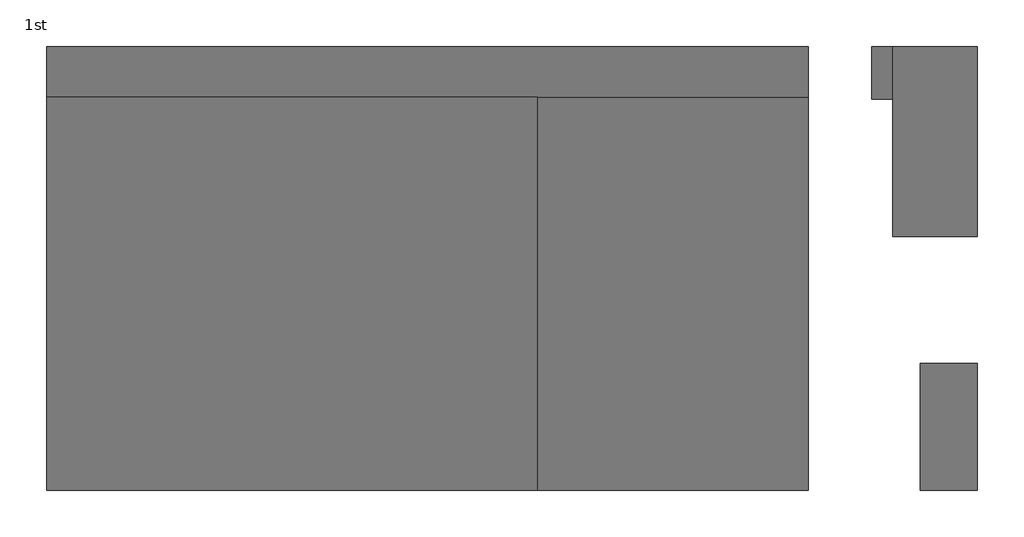
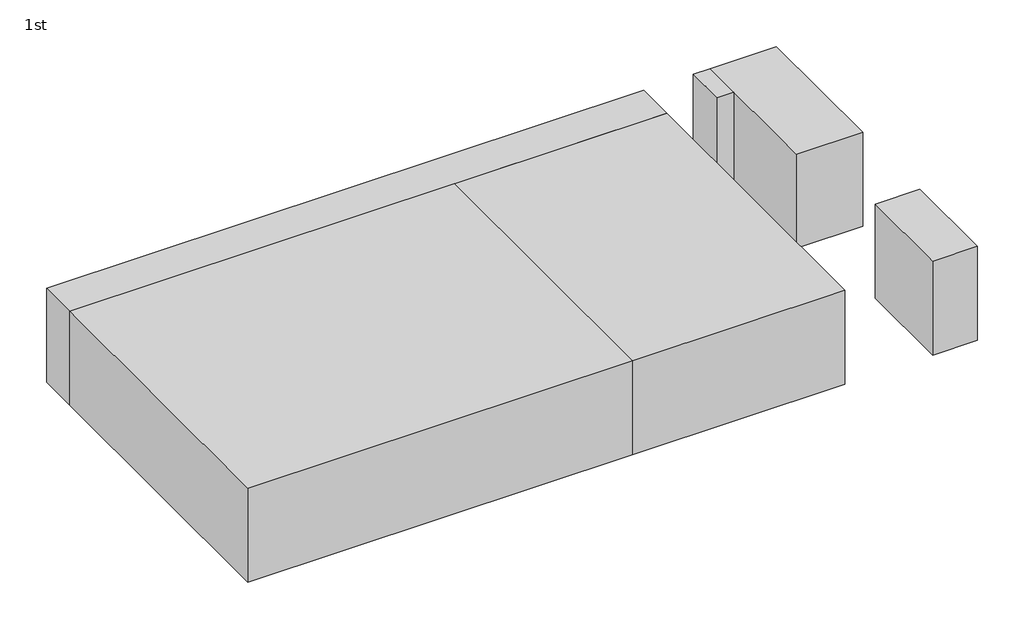
# One storey: 6 proxies.
"""IFC4 building model written with IfcOpenShell, lengths in millimetres."""

import ifcopenshell
import ifcopenshell.guid

model = None  # the IFC model being written
_history = None  # IfcOwnerHistory: only IFC2X3 demands one
_inside = {}  # id of a spatial element -> (the spatial element, [elements in it])
_under = {}  # id of a project, library or spatial element -> (it, [spatial elements below it])
_declared = {}  # id of a project -> (the project, [libraries it declares])
_typed = {}  # id of a type object -> (the type object, [elements of that type])
_made_of = {}  # id of a material, layer set ... -> (it, [elements and type objects made of it])


def new_model(schema):
    """Start an empty IFC model of exactly this schema.

    Asked for "IFC4X3", IfcOpenShell would pick the latest addendum, in which some entities
    have other attributes; the version numbers below select the first issue.
    IFC2X3 requires an IfcOwnerHistory on every rooted entity: one is made here for all.
    """
    global model, _history
    if schema == "IFC4X3":
        model = ifcopenshell.file(schema_version=(4, 3, 0, 0))
    else:
        model = ifcopenshell.file(schema=schema)
    _inside.clear()
    _under.clear()
    _declared.clear()
    _typed.clear()
    _made_of.clear()
    _history = None
    if model.schema == "IFC2X3":
        org = make("IfcOrganization", Name="unknown")
        user = make(
            "IfcPersonAndOrganization",
            ThePerson=make("IfcPerson", FamilyName="unknown"),
            TheOrganization=org,
        )
        app = make(
            "IfcApplication",
            ApplicationDeveloper=org,
            Version="unknown",
            ApplicationFullName="unknown",
            ApplicationIdentifier="unknown",
        )
        _history = make(
            "IfcOwnerHistory",
            OwningUser=user,
            OwningApplication=app,
            ChangeAction="ADDED",
            CreationDate=0,
        )
    return model


def make(cls, **values):
    """One entity of the class cls with the attributes given. An attribute that is None is left unset."""
    return model.create_entity(
        cls, **{name: value for name, value in values.items() if value is not None}
    )


def rooted(cls, **values):
    """An entity with a GlobalId (a new one), such as an element, a storey or a relation."""
    return make(cls, GlobalId=ifcopenshell.guid.new(), OwnerHistory=_history, **values)


def si_unit(unit_type, name, prefix=None):
    """IfcSIUnit, for example si_unit("LENGTHUNIT", "METRE", prefix="MILLI")."""
    return make("IfcSIUnit", UnitType=unit_type, Prefix=prefix, Name=name)


def assignment(units):
    """IfcUnitAssignment: the units of a project."""
    return None if units is None else make("IfcUnitAssignment", Units=units)


def point(xyz):
    """IfcCartesianPoint."""
    return None if xyz is None else make("IfcCartesianPoint", Coordinates=xyz)


def direction(xyz):
    """IfcDirection."""
    return None if xyz is None else make("IfcDirection", DirectionRatios=xyz)


def frame(location, z_axis=None, x_axis=None):
    """IfcAxis2Placement3D, a coordinate frame: its origin and axes. An axis left out is left unset."""
    return make(
        "IfcAxis2Placement3D",
        Location=point(location),
        Axis=direction(z_axis),
        RefDirection=direction(x_axis),
    )


def origin():
    """The frame at (0, 0, 0) with its axes left unset."""
    return frame((0.0, 0.0, 0.0))


def origin_with_axes():
    """The frame at (0, 0, 0) with the z axis (0, 0, 1) and the x axis (1, 0, 0) written out."""
    return frame((0.0, 0.0, 0.0), z_axis=(0.0, 0.0, 1.0), x_axis=(1.0, 0.0, 0.0))


def place(relative_to, where):
    """IfcLocalPlacement: puts the frame where relative to a parent placement (None: the world)."""
    return make(
        "IfcLocalPlacement", PlacementRelTo=relative_to, RelativePlacement=where
    )


def context(
    kind, dimensions, precision=None, world=None, true_north=None, identifier=None
):
    """IfcGeometricRepresentationContext, for example the 3D "Model" context."""
    return make(
        "IfcGeometricRepresentationContext",
        ContextIdentifier=identifier,
        ContextType=kind,
        CoordinateSpaceDimension=dimensions,
        Precision=precision,
        WorldCoordinateSystem=world,
        TrueNorth=true_north,
    )


def project(units=None, contexts=None):
    """IfcProject with its units and contexts."""
    return rooted(
        "IfcProject",
        Name="project",
        RepresentationContexts=contexts,
        UnitsInContext=assignment(units),
    )


def spatial(cls, under=None, at=None, **own):
    """A site, building, storey or space (cls), placed at a placement, below another one or the project."""
    s = rooted(cls, ObjectPlacement=at, **own)
    if under is not None:
        _under.setdefault(under.id(), (under, []))[1].append(s)
    return s


def polyline(points):
    """IfcPolyline through the points."""
    return make("IfcPolyline", Points=[point(p) for p in points])


def outline(outer, holes=None, kind="AREA"):
    """IfcArbitraryClosedProfileDef: a profile drawn as a closed curve; with holes, ...WithVoids."""
    if holes is None:
        return make("IfcArbitraryClosedProfileDef", ProfileType=kind, OuterCurve=outer)
    return make(
        "IfcArbitraryProfileDefWithVoids",
        ProfileType=kind,
        OuterCurve=outer,
        InnerCurves=holes,
    )


def extrude(swept, where, along, depth):
    """IfcExtrudedAreaSolid: the profile swept, set in the frame where, extruded along a direction by depth."""
    return make(
        "IfcExtrudedAreaSolid",
        SweptArea=swept,
        Position=where,
        ExtrudedDirection=direction(along),
        Depth=depth,
    )


def shape(context_of_items, identifier, shape_type, items):
    """IfcShapeRepresentation: the items that make up one representation, for example the "Body"."""
    return make(
        "IfcShapeRepresentation",
        ContextOfItems=context_of_items,
        RepresentationIdentifier=identifier,
        RepresentationType=shape_type,
        Items=items,
    )


def source(mapping_origin, context_of_items, identifier, shape_type, items):
    """IfcRepresentationMap: a shape defined once, which mapped items show again and again."""
    return make(
        "IfcRepresentationMap",
        MappingOrigin=mapping_origin,
        MappedRepresentation=shape(context_of_items, identifier, shape_type, items),
    )


def transform(
    local_origin,
    x_axis=None,
    y_axis=None,
    z_axis=None,
    scale=None,
    scale2=None,
    scale3=None,
    uniform=True,
):
    """IfcCartesianTransformationOperator3D, or its non-uniform kind. x_axis, y_axis, z_axis: its Axis1, 2, 3."""
    if uniform:
        return make(
            "IfcCartesianTransformationOperator3D",
            Axis1=direction(x_axis),
            Axis2=direction(y_axis),
            LocalOrigin=point(local_origin),
            Scale=scale,
            Axis3=direction(z_axis),
        )
    return make(
        "IfcCartesianTransformationOperator3DnonUniform",
        Axis1=direction(x_axis),
        Axis2=direction(y_axis),
        LocalOrigin=point(local_origin),
        Scale=scale,
        Axis3=direction(z_axis),
        Scale2=scale2,
        Scale3=scale3,
    )


def mapped(mapping_source, mapping_target):
    """IfcMappedItem: shows the shape of a source again, moved by a transform."""
    return make(
        "IfcMappedItem", MappingSource=mapping_source, MappingTarget=mapping_target
    )


def made_of(thing, what):
    """Note that an element or type object is made of a material, layer set ...; save() writes the relation."""
    if what is not None:
        _made_of.setdefault(what.id(), (what, []))[1].append(thing)
    return thing


def element(
    cls,
    number,
    at=None,
    inside=None,
    cuts=None,
    type_object=None,
    material=None,
    context=None,
    identifier="Body",
    shape_type=None,
    held_by="IfcProductDefinitionShape",
    body=None,
    shapes=None,
    **own,
):
    """One element of the class cls, such as IfcWall. Its Tag is "e" and its number.

    at: its placement. inside: the storey or other place that contains it. cuts: it is an
    opening in that element (IfcRelVoidsElement). A single representation is given by context,
    identifier, shape_type and body (its items); several are given by shapes. held_by: the class
    of the entity that holds the representations. save() writes the other relations.
    """
    e = rooted(cls, Tag="e%d" % number, ObjectPlacement=at, **own)
    if body is not None:
        shapes = [shape(context, identifier, shape_type, body)]
    if shapes is not None:
        e.Representation = make(held_by, Representations=shapes)
    if inside is not None:
        _inside.setdefault(inside.id(), (inside, []))[1].append(e)
    if cuts is not None:
        rooted(
            "IfcRelVoidsElement", RelatingBuildingElement=cuts, RelatedOpeningElement=e
        )
    if type_object is not None:
        _typed.setdefault(type_object.id(), (type_object, []))[1].append(e)
    return made_of(e, material)


def aggregate(whole, parts):
    """IfcRelAggregates: a whole, such as a stair, and the parts it consists of."""
    return rooted("IfcRelAggregates", RelatingObject=whole, RelatedObjects=parts)


def save(model, path):
    """Write the relations noted so far, then the file.

    IfcRelAggregates (storeys below a building ...), IfcRelContainedInSpatialStructure (elements
    in a storey), IfcRelDefinesByType, IfcRelAssociatesMaterial and IfcRelDeclares: one each for
    every whole, place, type object, material and project.
    """
    for whole, parts in _under.values():
        aggregate(whole, parts)
    for where, things in _inside.values():
        rooted(
            "IfcRelContainedInSpatialStructure",
            RelatedElements=things,
            RelatingStructure=where,
        )
    for kind, things in _typed.values():
        rooted("IfcRelDefinesByType", RelatedObjects=things, RelatingType=kind)
    for what, things in _made_of.values():
        rooted("IfcRelAssociatesMaterial", RelatedObjects=things, RelatingMaterial=what)
    for by, libraries in _declared.values():
        rooted("IfcRelDeclares", RelatingContext=by, RelatedDefinitions=libraries)
    model.write(path)


def space_planning_box_space_planning_box_29bcd6f9(model_context):
    return source(origin(), model_context, "Body", "SweptSolid", [
        extrude(outline(polyline([(2000.0, 4500.0), (2000.0, -4500.0), (-2000.0, -4500.0), (-2000.0, 4500.0), (2000.0, 4500.0)])), origin_with_axes(), (0.0, 0.0, 1.0), 6000.0),
    ])


def space_planning_box_space_planning_box_d82b1902(model_context):
    return source(origin(), model_context, "Body", "SweptSolid", [
        extrude(outline(polyline([(9300.0, 11600.0), (9300.0, -11600.0), (-9300.0, -11600.0), (-9300.0, 11600.0), (9300.0, 11600.0)])), origin_with_axes(), (0.0, 0.0, 1.0), 6000.0),
    ])


def space_planning_box_space_planning_box_21711933(model_context):
    return source(origin(), model_context, "Body", "SweptSolid", [
        extrude(outline(polyline([(6400.0, 9300.0), (6400.0, -9300.0), (-6400.0, -9300.0), (-6400.0, 9300.0), (6400.0, 9300.0)])), origin_with_axes(), (0.0, 0.0, 1.0), 6000.0),
    ])


def space_planning_box_space_planning_box_03d31222(model_context):
    return source(origin(), model_context, "Body", "SweptSolid", [
        extrude(outline(polyline([(1200.0, 18000.0), (1200.0, -18000.0), (-1200.0, -18000.0), (-1200.0, 18000.0), (1200.0, 18000.0)])), origin_with_axes(), (0.0, 0.0, 1.0), 6000.0),
    ])


def space_planning_box_space_planning_box_5634f436(model_context):
    return source(origin(), model_context, "Body", "SweptSolid", [
        extrude(outline(polyline([(1350.0, 3000.0), (1350.0, -3000.0), (-1350.0, -3000.0), (-1350.0, 3000.0), (1350.0, 3000.0)])), origin_with_axes(), (0.0, 0.0, 1.0), 6000.0),
    ])


def space_planning_box_space_planning_box_71e2440f(model_context):
    return source(origin(), model_context, "Body", "SweptSolid", [
        extrude(outline(polyline([(500.0, 1250.0), (500.0, -1250.0), (-500.0, -1250.0), (-500.0, 1250.0), (500.0, 1250.0)])), origin_with_axes(), (0.0, 0.0, 1.0), 6000.0),
    ])


model = new_model("IFC4")

# Units and contexts
model_context = context("Model", 3, world=origin())
ifc_project = project(units=[si_unit("LENGTHUNIT", "METRE", prefix="MILLI")], contexts=[model_context])

# Site, building, storey
site = spatial("IfcSite", under=ifc_project)
building = spatial("IfcBuilding", under=site)
storey = spatial("IfcBuildingStorey", under=building, Name="1st", Elevation=7000.0)

# Proxies
placement = place(None, origin())
space_planning_box_space_planning_box_shape = space_planning_box_space_planning_box_29bcd6f9(model_context)
element("IfcBuildingElementProxy", 1, Name="Space Planning Box : Space Planning Box", ObjectType="Space Planning Box : Space Planning Box", at=placement, inside=storey, context=model_context, shape_type="MappedRepresentation", body=[
    mapped(space_planning_box_space_planning_box_shape, transform((39700.0, 121200.0, 7000.0), x_axis=(1.0, 0.0, 0.0), y_axis=(0.0, 1.0, 0.0), z_axis=(0.0, 0.0, 1.0))),
])
space_planning_box_space_planning_box_2_shape = space_planning_box_space_planning_box_d82b1902(model_context)
element("IfcBuildingElementProxy", 2, Name="Space Planning Box : Space Planning Box", ObjectType="Space Planning Box : Space Planning Box", at=placement, inside=storey, context=model_context, shape_type="MappedRepresentation", body=[
    mapped(space_planning_box_space_planning_box_2_shape, transform((9300.0, 114000.0, 7000.0), x_axis=(0.0, -1.0, 0.0), y_axis=(1.0, 0.0, 0.0), z_axis=(0.0, 0.0, 1.0))),
])
space_planning_box_space_planning_box_3_shape = space_planning_box_space_planning_box_21711933(model_context)
element("IfcBuildingElementProxy", 3, Name="Space Planning Box : Space Planning Box", ObjectType="Space Planning Box : Space Planning Box", at=placement, inside=storey, context=model_context, shape_type="MappedRepresentation", body=[
    mapped(space_planning_box_space_planning_box_3_shape, transform((27300.0, 114000.0, 7000.0), x_axis=(1.0, 0.0, 0.0), y_axis=(0.0, 1.0, 0.0), z_axis=(0.0, 0.0, 1.0))),
])
space_planning_box_space_planning_box_4_shape = space_planning_box_space_planning_box_03d31222(model_context)
element("IfcBuildingElementProxy", 4, Name="Space Planning Box : Space Planning Box", ObjectType="Space Planning Box : Space Planning Box", at=placement, inside=storey, context=model_context, shape_type="MappedRepresentation", body=[
    mapped(space_planning_box_space_planning_box_4_shape, transform((15700.0, 124500.0, 7000.0), x_axis=(0.0, 1.0, 0.0), y_axis=(-1.0, 0.0, 0.0), z_axis=(0.0, 0.0, 1.0))),
])
space_planning_box_space_planning_box_5_shape = space_planning_box_space_planning_box_5634f436(model_context)
element("IfcBuildingElementProxy", 5, Name="Space Planning Box : Space Planning Box", ObjectType="Space Planning Box : Space Planning Box", at=placement, inside=storey, context=model_context, shape_type="MappedRepresentation", body=[
    mapped(space_planning_box_space_planning_box_5_shape, transform((40350.0, 107700.0, 7000.0), x_axis=(1.0, 0.0, 0.0), y_axis=(0.0, 1.0, 0.0), z_axis=(0.0, 0.0, 1.0))),
])
space_planning_box_space_planning_box_6_shape = space_planning_box_space_planning_box_71e2440f(model_context)
element("IfcBuildingElementProxy", 6, Name="Space Planning Box : Space Planning Box", ObjectType="Space Planning Box : Space Planning Box", at=placement, inside=storey, context=model_context, shape_type="MappedRepresentation", body=[
    mapped(space_planning_box_space_planning_box_6_shape, transform((37200.0, 124450.0, 7000.0), x_axis=(1.0, 0.0, 0.0), y_axis=(0.0, 1.0, 0.0), z_axis=(0.0, 0.0, 1.0))),
])

save(model, "model.ifc")

# Revit data of these elements
# Project information
#   Project Issue Date = "Issue Date"
#   Project Status = "Project Status"
#   Client Name = "Owner"
#   Project Address = "Enter address here"
#   Project Name = "Project Name"
#   Project Number = "Project Number"
# Type "Space Planning Box : Space Planning Box"
#   Type Comments = "..."
#   Room Name [instance default] = "?"
#   Assembly Code = "..."
#   Width [instance default] = 1524 mm
#   Program Area [instance default] = 0 m²
#   Length [instance default] = 1524 mm
#   Height [instance default] = 1524 mm
#   Area [instance default] = 2.32258 m²
#   Fill Color [instance default] = Cyan
#   Default Elevation = 0
# Element 1 (IfcBuildingElementProxy, "Space Planning Box : Space Planning Box")
#   Room Name = "Stairway"
#   Width = 4000 mm
#   Program Area = 36 m²
#   Length = 9000 mm
#   Height = 6000 mm
#   Area = 36 m²
#   Fill Color = Lavender
#   Phase Created = New Construction
#   Materials on its faces: "Lavender"
# Element 2 (IfcBuildingElementProxy, "Space Planning Box : Space Planning Box")
#   Room Name = "Electronic Room"
#   Width = 18600 mm
#   Program Area = 431.52 m²
#   Length = 23200 mm
#   Height = 6000 mm
#   Area = 431.52 m²
#   Fill Color = Lime
#   Phase Created = New Construction
#   Materials on its faces: "Lime"
# Element 3 (IfcBuildingElementProxy, "Space Planning Box : Space Planning Box")
#   Room Name = "Electrical Room"
#   Width = 12800 mm
#   Program Area = 238.08 m²
#   Length = 18600 mm
#   Height = 6000 mm
#   Area = 238.08 m²
#   Fill Color = Blue
#   Phase Created = New Construction
#   Materials on its faces: "Blue"
# Element 4 (IfcBuildingElementProxy, "Space Planning Box : Space Planning Box")
#   Room Name = "Corridor"
#   Width = 2400 mm
#   Program Area = 86.4 m²
#   Length = 36000 mm
#   Height = 6000 mm
#   Area = 86.4 m²
#   Fill Color = Lavender
#   Phase Created = New Construction
#   Materials on its faces: "Lavender"
# Element 5 (IfcBuildingElementProxy, "Space Planning Box : Space Planning Box")
#   Room Name = "Duct Shaft"
#   Width = 2700 mm
#   Program Area = 16.2 m²
#   Length = 6000 mm
#   Height = 6000 mm
#   Area = 16.2 m²
#   Fill Color = Pink
#   Phase Created = New Construction
#   Materials on its faces: "Pink"
# Element 6 (IfcBuildingElementProxy, "Space Planning Box : Space Planning Box")
#   Room Name = "Pipe Shaft"
#   Width = 1000 mm
#   Program Area = 2.5 m²
#   Length = 2500 mm
#   Height = 6000 mm
#   Area = 2.5 m²
#   Fill Color = Pink
#   Phase Created = New Construction
#   Materials on its faces: "Pink"
# Materials
#   "Cyan": class "Generic", colour RGB 0 255 255, transparency 0.2, Cost = 0
#   "Lavender": class "Generic", colour RGB 186 85 211, transparency 0.2, Cost = 0
#   "Lime": class "Generic", colour RGB 0 255 0, transparency 0.2, Cost = 0
#   "Blue": class "Generic", colour RGB 0 0 255, transparency 0.2, Cost = 0
#   "Pink": class "Generic", colour RGB 255 105 180, transparency 0.2, Cost = 0
